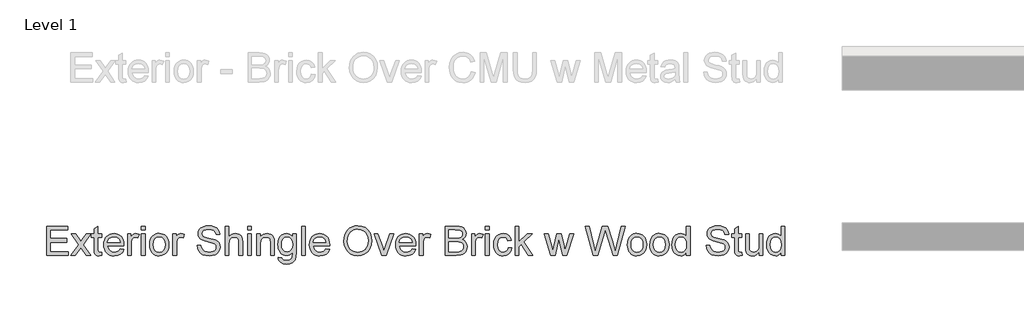
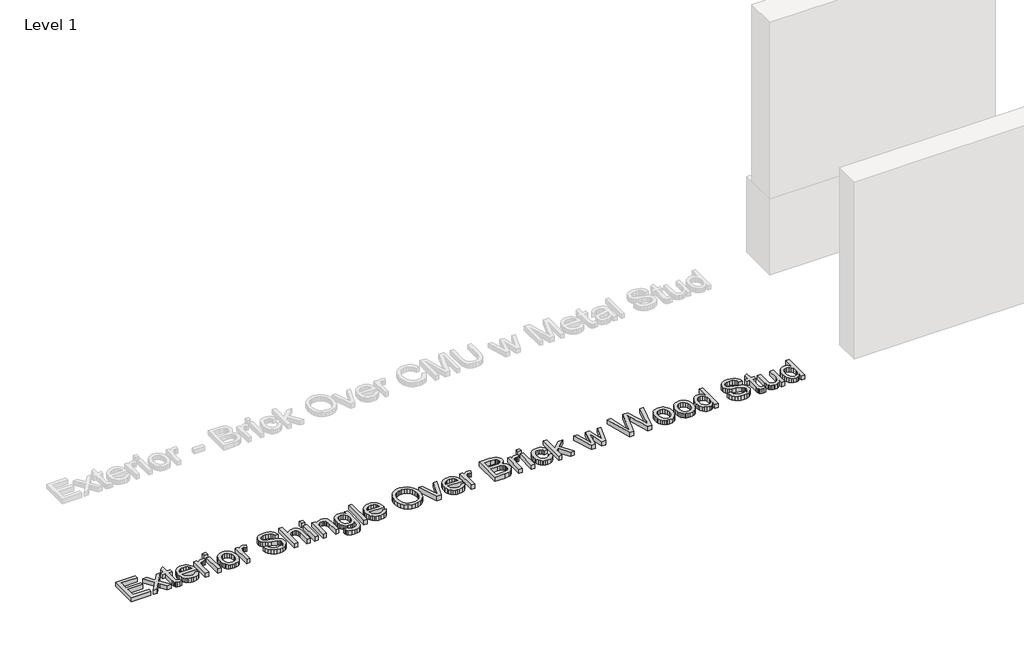
# One storey, part 38 of 42: 1 proxy.
"""IFC4 building model written with IfcOpenShell, lengths in millimetres."""

from ifc_helpers import new_model, si_unit, origin, origin_with_axes, place, context, project, spatial, polyline, outline, extrude, element, save

model = new_model("IFC4")

# Units and contexts
model_context = context("Model", 3, world=origin())
ifc_project = project(units=[si_unit("LENGTHUNIT", "METRE", prefix="MILLI")], contexts=[model_context])

# Site, building, storey
site = spatial("IfcSite", under=ifc_project)
building = spatial("IfcBuilding", under=site)
storey = spatial("IfcBuildingStorey", under=building, Name="Level 1", Elevation=0.0)

# Proxy
placement = place(None, origin())
element("IfcBuildingElementProxy", 1, Name="8\" Arial", ObjectType="8\" Arial", at=placement, inside=storey, context=model_context, shape_type="SweptSolid", body=[
    extrude(outline(polyline([(27228.7881133, 13210.6462247), (27228.7881133, 13515.2133187), (27447.6957121, 13515.2133187), (27447.6957121, 13477.142432), (27266.859, 13477.142432), (27266.859, 13386.7240759), (27438.1779905, 13386.7240759), (27438.1779905, 13348.6531892), (27266.859, 13348.6531892), (27266.859, 13248.7171114), (27452.454573, 13248.7171114), (27452.454573, 13210.6462247), (27228.7881133, 13210.6462247)])), origin_with_axes(), (0.0, 0.0, 1.0), 50.8),
    extrude(outline(polyline([(27481.0077381, 13210.6462247), (27562.3545156, 13323.0743121), (27485.7665989, 13434.3126844), (27531.5706345, 13434.3126844), (27568.5261633, 13380.7754999), (27585.7770338, 13355.4940516), (27600.7228312, 13376.1653534), (27642.8090068, 13434.3126844), (27688.6130424, 13434.3126844), (27608.1585513, 13323.0743121), (27685.6387544, 13210.6462247), (27639.8347188, 13210.6462247), (27593.2127539, 13278.2369201), (27584.6616758, 13290.5802154), (27526.8117737, 13210.6462247), (27481.0077381, 13210.6462247)])), origin_with_axes(), (0.0, 0.0, 1.0), 50.8),
    extrude(outline(polyline([(27799.8514147, 13242.3967494), (27804.6102755, 13209.5308667), (27776.1314676, 13205.8873638), (27757.8581856, 13207.4674543), (27744.2322285, 13212.2077259), (27734.602971, 13219.5133208), (27728.3197876, 13228.7893816), (27724.8621778, 13244.7204119), (27723.7096411, 13271.9909152), (27723.7096411, 13396.2417976), (27695.1564761, 13396.2417976), (27695.1564761, 13434.3126844), (27723.7096411, 13434.3126844), (27723.7096411, 13488.6677981), (27761.7805279, 13511.0493155), (27761.7805279, 13434.3126844), (27799.8514147, 13434.3126844), (27799.8514147, 13396.2417976), (27761.7805279, 13396.2417976), (27761.7805279, 13273.1062732), (27763.7881723, 13253.4759723), (27770.2944274, 13246.523574), (27783.2697589, 13243.9582506), (27799.8514147, 13242.3967494)])), origin_with_axes(), (0.0, 0.0, 1.0), 50.8),
    extrude(outline(polyline([(27994.5185661, 13277.2702765), (28031.8458808, 13272.5114156), (28018.3965222, 13244.3858045), (27996.9351751, 13223.361306), (27967.9451615, 13210.2558494), (27931.9098031, 13205.8873638), (27908.2874499, 13207.7718541), (27887.2397148, 13213.425325), (27868.7665977, 13222.8477766), (27852.8680988, 13236.0392087), (27840.0833076, 13252.6324828), (27830.9513139, 13272.2604601), (27825.4721176, 13294.9231407), (27823.6457189, 13320.6205245), (27825.4907069, 13347.1892818), (27831.0256711, 13370.6071527), (27840.2506113, 13390.8741372), (27853.1655276, 13407.9902353), (27869.0222006, 13421.5883084), (27887.0724111, 13431.3012177), (27907.316159, 13437.1289633), (27929.7534443, 13439.0715452), (27951.4680706, 13437.1336107), (27971.1053425, 13431.319807), (27988.6652602, 13421.6301343), (28004.1478236, 13408.0645925), (28016.786224, 13390.985673), (28025.8136529, 13370.7558671), (28031.2301103, 13347.3751748), (28033.0355961, 13320.8435961), (28032.8125245, 13310.5823024), (27861.7166056, 13310.5823024), (27868.3065126, 13282.0849052), (27883.6148013, 13261.1347639), (27905.7081845, 13248.2523789), (27932.6533751, 13243.9582506), (27952.9157123, 13245.9473057), (27969.9806899, 13251.9144711), (27983.8483078, 13262.2315326), (27994.5185661, 13277.2702765)]), holes=[polyline([(27861.7166056, 13348.6531892), (27994.9647093, 13348.6531892), (27989.8154732, 13368.766812), (27979.7214832, 13383.1549303), (27957.5258587, 13396.5392264), (27929.6047299, 13401.0006585), (27903.942201, 13397.4408075), (27882.7225148, 13386.7612545), (27867.9719052, 13370.1145362), (27861.7166056, 13348.6531892)])]), origin_with_axes(), (0.0, 0.0, 1.0), 50.8),
    extrude(outline(polyline([(28071.1064828, 13210.6462247), (28071.1064828, 13434.3126844), (28104.4185087, 13434.3126844), (28104.4185087, 13401.2237301), (28116.7246254, 13420.4078878), (28128.0640986, 13431.7101823), (28139.4407503, 13437.2312045), (28151.8584028, 13439.0715452), (28170.819489, 13436.1344358), (28190.0780039, 13427.3231075), (28177.3629226, 13393.1931524), (28163.9786265, 13399.0487819), (28150.5943304, 13401.0006585), (28139.2269733, 13399.1231391), (28129.0679208, 13393.4905812), (28120.8607447, 13384.5305385), (28115.3490172, 13372.670565), (28110.7202815, 13351.4044056), (28109.1773696, 13328.204959), (28109.1773696, 13210.6462247), (28071.1064828, 13210.6462247)])), origin_with_axes(), (0.0, 0.0, 1.0), 50.8),
    extrude(outline(polyline([(28213.8723082, 13477.142432), (28213.8723082, 13515.2133187), (28251.9431949, 13515.2133187), (28251.9431949, 13477.142432), (28213.8723082, 13477.142432)])), origin_with_axes(), (0.0, 0.0, 1.0), 50.8),
    extrude(outline(polyline([(28213.8723082, 13210.6462247), (28213.8723082, 13434.3126844), (28251.9431949, 13434.3126844), (28251.9431949, 13210.6462247), (28213.8723082, 13210.6462247)])), origin_with_axes(), (0.0, 0.0, 1.0), 50.8),
    extrude(outline(polyline([(28299.5318034, 13322.4794545), (28301.5905684, 13351.4462315), (28307.7668633, 13376.4070143), (28318.0606883, 13397.3618029), (28332.4720433, 13414.3105974), (28346.9809921, 13425.1435121), (28362.9956742, 13432.8813083), (28380.5160896, 13437.523986), (28399.5422383, 13439.0715452), (28420.5458238, 13437.1870549), (28439.5371176, 13431.533584), (28456.5161197, 13422.1111325), (28471.48283, 13408.9197003), (28483.6983239, 13392.4054308), (28492.4236766, 13373.014467), (28497.6588883, 13350.7468091), (28499.4039589, 13325.6024569), (28496.318135, 13287.1411949), (28487.0606635, 13257.8630471), (28471.9010892, 13235.9369675), (28451.108957, 13219.5319101), (28426.4130717, 13209.2985004), (28399.5422383, 13205.8873638), (28378.2319293, 13207.7648831), (28359.0640372, 13213.3974411), (28342.0385619, 13222.7850377), (28327.1555034, 13235.9276729), (28315.0701347, 13252.6022752), (28306.4377284, 13272.5857728), (28301.2582846, 13295.878166), (28299.5318034, 13322.4794545)]), holes=[polyline([(28337.6026901, 13322.5538117), (28342.0083543, 13288.0985438), (28355.2253467, 13263.551373), (28375.1158979, 13248.8565312), (28399.5422383, 13243.9582506), (28423.8570429, 13248.8844151), (28443.7104155, 13263.6629088), (28456.927408, 13288.5353924), (28461.3330721, 13323.7435269), (28456.899524, 13357.1949726), (28443.5988797, 13381.4075361), (28423.7176232, 13396.1023779), (28399.5422383, 13401.0006585), (28375.1158979, 13396.1209672), (28355.2253467, 13381.4818933), (28342.0083543, 13356.9904903), (28337.6026901, 13322.5538117)])]), origin_with_axes(), (0.0, 0.0, 1.0), 50.8),
    extrude(outline(polyline([(28542.2337065, 13210.6462247), (28542.2337065, 13434.3126844), (28575.5457324, 13434.3126844), (28575.5457324, 13401.2237301), (28587.8518491, 13420.4078878), (28599.1913222, 13431.7101823), (28610.5679739, 13437.2312045), (28622.9856264, 13439.0715452), (28641.9467126, 13436.1344358), (28661.2052276, 13427.3231075), (28648.4901463, 13393.1931524), (28635.1058501, 13399.0487819), (28621.721554, 13401.0006585), (28610.3541969, 13399.1231391), (28600.1951444, 13393.4905812), (28591.9879684, 13384.5305385), (28586.4762409, 13372.670565), (28581.8475051, 13351.4044056), (28580.3045932, 13328.204959), (28580.3045932, 13210.6462247), (28542.2337065, 13210.6462247)])), origin_with_axes(), (0.0, 0.0, 1.0), 50.8),
    extrude(outline(polyline([(28794.4533312, 13315.3411632), (28832.524218, 13315.3411632), (28836.8927035, 13294.2144236), (28844.7931561, 13277.2330979), (28857.1178621, 13263.7558553), (28874.759108, 13253.1413649), (28896.3226962, 13246.2540291), (28920.4144292, 13243.9582506), (28941.6248207, 13245.6963501), (28960.1955316, 13250.9106488), (28975.2435701, 13259.1642981), (28985.8859444, 13270.0204494), (28992.2156011, 13282.4845752), (28994.3254867, 13295.5621479), (28992.7453962, 13308.3051131), (28988.0051247, 13319.3192735), (28978.3758672, 13328.7161647), (28962.1288188, 13336.6073226), (28906.6955257, 13351.1441554), (28870.3069706, 13360.7641182), (28847.0238721, 13369.9193486), (28828.0720806, 13382.7273764), (28814.6413112, 13398.249442), (28806.6386175, 13416.1509381), (28803.9710529, 13436.0972572), (28807.2706537, 13458.3951227), (28817.169456, 13479.187255), (28833.4072097, 13496.8099116), (28855.7236646, 13509.5993501), (28882.5108462, 13517.3789722), (28912.1607799, 13519.9721796), (28944.2830906, 13517.2581417), (28972.3901125, 13509.1160283), (28995.4780233, 13495.7131428), (29012.5430009, 13477.2167892), (29023.3433843, 13454.7795039), (29027.6375126, 13429.5538235), (28989.5666259, 13429.5538235), (28982.577049, 13452.2699483), (28968.0030377, 13468.6657111), (28945.231145, 13478.5923974), (28913.647924, 13481.9012928), (28881.3211309, 13478.629576), (28859.1440958, 13468.8144255), (28846.3174787, 13454.3705393), (28842.0419397, 13437.2126152), (28845.0719956, 13422.582836), (28854.1621634, 13410.8158089), (28875.6513944, 13400.294265), (28916.3247832, 13389.5496495), (28958.299423, 13379.3441238), (28983.692407, 13370.439849), (29005.395415, 13356.6279989), (29020.5364, 13339.5816107), (29029.4313801, 13319.4865772), (29032.3963735, 13296.5287915), (29028.9852369, 13273.0598), (29018.7518271, 13250.985006), (29002.1144035, 13231.9867413), (28979.4912252, 13217.7473373), (28952.2857844, 13208.8523572), (28921.9015732, 13205.8873638), (28884.6021424, 13209.0847234), (28853.9019132, 13218.6768023), (28829.4476888, 13234.7007791), (28810.8862726, 13257.1938323), (28798.9705312, 13284.5944608), (28794.4533312, 13315.3411632)])), origin_with_axes(), (0.0, 0.0, 1.0), 50.8),
    extrude(outline(polyline([(29084.7438428, 13210.6462247), (29084.7438428, 13515.2133187), (29122.8147295, 13515.2133187), (29122.8147295, 13403.2313745), (29136.7985306, 13418.9114492), (29152.5018419, 13430.1115025), (29169.9246635, 13436.8315345), (29189.0669953, 13439.0715452), (29212.0619597, 13436.6270522), (29231.8223858, 13429.2935733), (29247.38163, 13417.6473768), (29257.7730488, 13402.2647309), (29263.6286783, 13381.1286966), (29265.5805549, 13352.2223348), (29265.5805549, 13210.6462247), (29227.5096681, 13210.6462247), (29227.5096681, 13348.2814032), (29224.4796122, 13372.112886), (29215.3894444, 13388.4342915), (29200.7410759, 13397.8590667), (29181.0364177, 13401.0006585), (29164.9473784, 13398.8814782), (29149.843572, 13392.5239376), (29137.332973, 13382.5414834), (29129.0235558, 13369.5475626), (29124.3669361, 13352.2781027), (29122.8147295, 13329.4690314), (29122.8147295, 13210.6462247), (29084.7438428, 13210.6462247)])), origin_with_axes(), (0.0, 0.0, 1.0), 50.8),
    extrude(outline(polyline([(29317.9280242, 13210.6462247), (29317.9280242, 13434.3126844), (29355.9989109, 13434.3126844), (29355.9989109, 13210.6462247), (29317.9280242, 13210.6462247)])), origin_with_axes(), (0.0, 0.0, 1.0), 50.8),
    extrude(outline(polyline([(29317.9280242, 13477.142432), (29317.9280242, 13515.2133187), (29355.9989109, 13515.2133187), (29355.9989109, 13477.142432), (29317.9280242, 13477.142432)])), origin_with_axes(), (0.0, 0.0, 1.0), 50.8),
    extrude(outline(polyline([(29413.1052411, 13210.6462247), (29413.1052411, 13434.3126844), (29451.1761278, 13434.3126844), (29451.1761278, 13403.0826601), (29464.4024149, 13418.8277973), (29480.2869719, 13430.0743239), (29498.8297988, 13436.8222399), (29520.0308957, 13439.0715452), (29538.7967942, 13437.2590884), (29555.9826022, 13431.8217181), (29570.3149526, 13423.4379438), (29580.5204784, 13412.7862748), (29591.9343087, 13384.7907887), (29593.9419532, 13347.9839744), (29593.9419532, 13210.6462247), (29555.8710664, 13210.6462247), (29555.8710664, 13342.8533275), (29551.4839916, 13376.5371394), (29545.4145851, 13386.5660669), (29535.9805152, 13394.345689), (29523.8881755, 13399.3369161), (29509.8439592, 13401.0006585), (29487.5460936, 13397.2642091), (29468.5385342, 13386.0548611), (29460.9424814, 13376.9042781), (29455.5167294, 13364.3983264), (29451.1761278, 13329.320317), (29451.1761278, 13210.6462247), (29413.1052411, 13210.6462247)])), origin_with_axes(), (0.0, 0.0, 1.0), 50.8),
    extrude(outline(polyline([(29636.7717008, 13191.6107813), (29674.8425875, 13186.8519204), (29679.0437694, 13174.9547683), (29687.1858828, 13166.7754762), (29703.1912703, 13160.4179356), (29724.1414116, 13158.2987554), (29746.4857504, 13160.6967751), (29763.1045848, 13167.8908343), (29774.6299509, 13179.4162004), (29781.6938849, 13194.8081409), (29784.296387, 13239.1993897), (29771.6277789, 13226.70738), (29757.4906161, 13217.7845159), (29741.8848986, 13212.4307975), (29724.8106264, 13210.6462247), (29703.937166, 13212.723579), (29685.5593191, 13218.9556418), (29669.6770857, 13229.3424133), (29656.2904659, 13243.8838934), (29645.6690046, 13261.3299516), (29638.0822464, 13280.4304575), (29633.5301915, 13301.1854112), (29632.0128399, 13323.5948125), (29634.7361724, 13354.3322204), (29642.9061698, 13382.5972513), (29656.234698, 13406.5495646), (29674.4336229, 13424.3488195), (29696.8802029, 13435.3908638), (29722.9516964, 13439.0715452), (29740.7555986, 13436.9895436), (29756.9143478, 13430.7435387), (29771.4279439, 13420.3335306), (29784.296387, 13405.7595193), (29784.296387, 13434.3126844), (29822.3672737, 13434.3126844), (29822.3672737, 13241.2070341), (29819.7647717, 13196.6205977), (29811.9572656, 13167.2587981), (29798.5079069, 13147.7865061), (29778.9798471, 13132.8685927), (29753.80064, 13123.3880496), (29723.3978396, 13120.2278686), (29687.9759281, 13124.680006), (29660.0826832, 13138.0364182), (29649.5774049, 13148.063022), (29642.1904818, 13160.3342837), (29637.9219137, 13174.8502035), (29636.7717008, 13191.6107813)]), holes=[polyline([(29670.0837267, 13326.1973145), (29674.1454888, 13291.2773142), (29686.330775, 13267.269233), (29704.6505304, 13253.3551418), (29727.1156996, 13248.7171114), (29749.4135652, 13253.3272579), (29767.826267, 13267.1576972), (29780.178857, 13290.8590549), (29784.296387, 13325.0819565), (29780.0580265, 13358.087259), (29767.3429452, 13381.8536793), (29748.6606985, 13396.2139137), (29726.520842, 13401.0006585), (29704.7806555, 13396.2882709), (29686.5538466, 13382.1511081), (29674.2012567, 13358.7378845), (29670.0837267, 13326.1973145)])]), origin_with_axes(), (0.0, 0.0, 1.0), 50.8),
    extrude(outline(polyline([(29879.4736038, 13210.6462247), (29879.4736038, 13515.2133187), (29917.5444906, 13515.2133187), (29917.5444906, 13210.6462247), (29879.4736038, 13210.6462247)])), origin_with_axes(), (0.0, 0.0, 1.0), 50.8),
    extrude(outline(polyline([(30131.2470854, 13277.2702765), (30168.5744002, 13272.5114156), (30155.1250415, 13244.3858045), (30133.6636944, 13223.361306), (30104.6736808, 13210.2558494), (30068.6383224, 13205.8873638), (30045.0159692, 13207.7718541), (30023.9682341, 13213.425325), (30005.4951171, 13222.8477766), (29989.5966181, 13236.0392087), (29976.8118269, 13252.6324828), (29967.6798332, 13272.2604601), (29962.200637, 13294.9231407), (29960.3742382, 13320.6205245), (29962.2192263, 13347.1892818), (29967.7541904, 13370.6071527), (29976.9791306, 13390.8741372), (29989.8940469, 13407.9902353), (30005.7507199, 13421.5883084), (30023.8009304, 13431.3012177), (30044.0446783, 13437.1289633), (30066.4819636, 13439.0715452), (30088.1965899, 13437.1336107), (30107.8338619, 13431.319807), (30125.3937795, 13421.6301343), (30140.8763429, 13408.0645925), (30153.5147434, 13390.985673), (30162.5421723, 13370.7558671), (30167.9586296, 13347.3751748), (30169.7641154, 13320.8435961), (30169.5410438, 13310.5823024), (29998.445125, 13310.5823024), (30005.0350319, 13282.0849052), (30020.3433206, 13261.1347639), (30042.4367038, 13248.2523789), (30069.3818944, 13243.9582506), (30089.6442316, 13245.9473057), (30106.7092092, 13251.9144711), (30120.5768271, 13262.2315326), (30131.2470854, 13277.2702765)]), holes=[polyline([(29998.445125, 13348.6531892), (30131.6932286, 13348.6531892), (30126.5439925, 13368.766812), (30116.4500025, 13383.1549303), (30094.2543781, 13396.5392264), (30066.3332492, 13401.0006585), (30040.6707203, 13397.4408075), (30019.4510342, 13386.7612545), (30004.7004245, 13370.1145362), (29998.445125, 13348.6531892)])]), origin_with_axes(), (0.0, 0.0, 1.0), 50.8),
    extrude(outline(polyline([(30317.2888016, 13358.9144829), (30319.826241, 13394.6384705), (30327.4385595, 13426.2635174), (30340.1257568, 13453.7896236), (30357.8878332, 13477.2167892), (30379.660551, 13495.9222725), (30404.3796729, 13509.283332), (30432.0451989, 13517.2999677), (30462.6571289, 13519.9721796), (30502.605535, 13514.9530685), (30538.4271165, 13499.8957354), (30568.1699967, 13475.8597703), (30589.8822993, 13443.9047633), (30603.1550597, 13405.5736263), (30607.5793131, 13362.4092713), (30602.9226934, 13318.668648), (30588.9528343, 13279.7984213), (30566.4411918, 13247.7876464), (30536.1592218, 13224.6253784), (30500.6443638, 13210.5718675), (30462.4340573, 13205.8873638), (30421.8722044, 13211.0644839), (30385.8461406, 13226.5958442), (30356.1776175, 13251.0779525), (30334.6883865, 13283.1073167), (30321.6386978, 13319.9606043), (30317.2888016, 13358.9144829)]), holes=[polyline([(30355.3596883, 13358.5426969), (30357.2627679, 13333.3030745), (30362.9720068, 13310.8983205), (30372.4874048, 13291.3284347), (30385.808962, 13274.5934173), (30402.0025661, 13261.1905318), (30420.1341048, 13251.6170422), (30440.203578, 13245.8729485), (30462.2109857, 13243.9582506), (30484.5948268, 13245.8915378), (30504.9013136, 13251.6913994), (30523.1304461, 13261.3578355), (30539.2822243, 13274.8908461), (30552.5061877, 13291.9790603), (30561.9518758, 13312.3111073), (30567.6192887, 13335.8869873), (30569.5084263, 13362.7067001), (30566.2738881, 13396.4091013), (30556.5702734, 13425.5385347), (30540.6485378, 13449.3607229), (30518.7596369, 13467.1413885), (30492.353536, 13478.2113167), (30462.8802005, 13481.9012928), (30441.6372778, 13480.123691), (30421.9279723, 13474.7908855), (30403.752284, 13465.9028764), (30387.110213, 13453.4596635), (30373.2193585, 13436.8617422), (30363.2973195, 13415.5096072), (30357.3440961, 13389.4032588), (30355.3596883, 13358.5426969)])]), origin_with_axes(), (0.0, 0.0, 1.0), 50.8),
    extrude(outline(polyline([(30710.0435357, 13210.6462247), (30631.3736173, 13434.3126844), (30671.6752201, 13434.3126844), (30719.3381858, 13300.3210087), (30733.6891255, 13255.2605451), (30747.7426364, 13297.7928639), (30795.7030309, 13434.3126844), (30836.0046337, 13434.3126844), (30758.3013589, 13210.6462247), (30710.0435357, 13210.6462247)])), origin_with_axes(), (0.0, 0.0, 1.0), 50.8),
    extrude(outline(polyline([(31025.9129242, 13277.2702765), (31063.240239, 13272.5114156), (31049.7908803, 13244.3858045), (31028.3295333, 13223.361306), (30999.3395196, 13210.2558494), (30963.3041613, 13205.8873638), (30939.6818081, 13207.7718541), (30918.6340729, 13213.425325), (30900.1609559, 13222.8477766), (30884.2624569, 13236.0392087), (30871.4776657, 13252.6324828), (30862.345672, 13272.2604601), (30856.8664758, 13294.9231407), (30855.040077, 13320.6205245), (30856.8850651, 13347.1892818), (30862.4200292, 13370.6071527), (30871.6449694, 13390.8741372), (30884.5598857, 13407.9902353), (30900.4165588, 13421.5883084), (30918.4667692, 13431.3012177), (30938.7105171, 13437.1289633), (30961.1478024, 13439.0715452), (30982.8624287, 13437.1336107), (31002.4997007, 13431.319807), (31020.0596184, 13421.6301343), (31035.5421817, 13408.0645925), (31048.1805822, 13390.985673), (31057.2080111, 13370.7558671), (31062.6244684, 13347.3751748), (31064.4299542, 13320.8435961), (31064.2068826, 13310.5823024), (30893.1109638, 13310.5823024), (30899.7008707, 13282.0849052), (30915.0091594, 13261.1347639), (30937.1025427, 13248.2523789), (30964.0477333, 13243.9582506), (30984.3100705, 13245.9473057), (31001.375048, 13251.9144711), (31015.2426659, 13262.2315326), (31025.9129242, 13277.2702765)]), holes=[polyline([(30893.1109638, 13348.6531892), (31026.3590675, 13348.6531892), (31021.2098313, 13368.766812), (31011.1158413, 13383.1549303), (30988.9202169, 13396.5392264), (30960.999088, 13401.0006585), (30935.3365591, 13397.4408075), (30914.116873, 13386.7612545), (30899.3662633, 13370.1145362), (30893.1109638, 13348.6531892)])]), origin_with_axes(), (0.0, 0.0, 1.0), 50.8),
    extrude(outline(polyline([(31102.500841, 13210.6462247), (31102.500841, 13434.3126844), (31135.8128669, 13434.3126844), (31135.8128669, 13401.2237301), (31148.1189836, 13420.4078878), (31159.4584567, 13431.7101823), (31170.8351084, 13437.2312045), (31183.2527609, 13439.0715452), (31202.2138471, 13436.1344358), (31221.4723621, 13427.3231075), (31208.7572808, 13393.1931524), (31195.3729846, 13399.0487819), (31181.9886885, 13401.0006585), (31170.6213315, 13399.1231391), (31160.4622789, 13393.4905812), (31152.2551029, 13384.5305385), (31146.7433754, 13372.670565), (31142.1146396, 13351.4044056), (31140.5717277, 13328.204959), (31140.5717277, 13210.6462247), (31102.500841, 13210.6462247)])), origin_with_axes(), (0.0, 0.0, 1.0), 50.8),
    extrude(outline(polyline([(31368.9970483, 13210.6462247), (31368.9970483, 13515.2133187), (31485.217353, 13515.2133187), (31517.1816546, 13512.9733081), (31542.1377901, 13506.253276), (31561.26618, 13494.885919), (31575.7472448, 13478.7039332), (31584.8652966, 13459.6684898), (31587.9046471, 13439.74076), (31585.3486184, 13421.4024154), (31577.680532, 13404.1608395), (31564.8446203, 13389.0756224), (31546.7851152, 13377.2063542), (31568.357998, 13365.9412383), (31584.2983229, 13348.8019036), (31594.1413573, 13326.9222973), (31597.4223688, 13301.4363667), (31595.1823582, 13280.1980913), (31588.4623261, 13260.5027277), (31578.4333987, 13243.7537683), (31566.2667017, 13231.3547051), (31551.3673776, 13222.3760731), (31533.1405688, 13215.8884073), (31484.3250666, 13210.6462247), (31368.9970483, 13210.6462247)]), holes=[polyline([(31407.067935, 13391.4829368), (31476.5919177, 13391.4829368), (31517.1909493, 13394.7546536), (31531.4024693, 13400.3965062), (31541.6172897, 13408.8453431), (31547.7796427, 13419.9710393), (31549.8337604, 13433.6434696), (31547.9190625, 13446.9162299), (31542.1749687, 13458.4787746), (31532.8617293, 13467.5038798), (31520.2395945, 13473.1643217), (31471.3125564, 13477.142432), (31407.067935, 13477.142432), (31407.067935, 13391.4829368)]), polyline([(31407.067935, 13248.7171114), (31485.1429958, 13248.7171114), (31513.398732, 13250.2042554), (31537.3045721, 13258.4950833), (31553.1426558, 13275.4113465), (31557.7992755, 13287.3642665), (31559.3514821, 13301.0645807), (31557.5297307, 13316.9770217), (31552.0644764, 13330.6587466), (31542.5188708, 13341.3568888), (31528.4560652, 13348.3185818), (31508.53763, 13352.1386829), (31481.4251357, 13353.41205), (31407.067935, 13353.41205), (31407.067935, 13248.7171114)])]), origin_with_axes(), (0.0, 0.0, 1.0), 50.8),
    extrude(outline(polyline([(31645.0109773, 13210.6462247), (31645.0109773, 13434.3126844), (31678.3230032, 13434.3126844), (31678.3230032, 13401.2237301), (31690.6291199, 13420.4078878), (31701.968593, 13431.7101823), (31713.3452447, 13437.2312045), (31725.7628972, 13439.0715452), (31744.7239834, 13436.1344358), (31763.9824984, 13427.3231075), (31751.2674171, 13393.1931524), (31737.883121, 13399.0487819), (31724.4988248, 13401.0006585), (31713.1314678, 13399.1231391), (31702.9724152, 13393.4905812), (31694.7652392, 13384.5305385), (31689.2535117, 13372.670565), (31684.6247759, 13351.4044056), (31683.081864, 13328.204959), (31683.081864, 13210.6462247), (31645.0109773, 13210.6462247)])), origin_with_axes(), (0.0, 0.0, 1.0), 50.8),
    extrude(outline(polyline([(31787.7768026, 13477.142432), (31787.7768026, 13515.2133187), (31825.8476894, 13515.2133187), (31825.8476894, 13477.142432), (31787.7768026, 13477.142432)])), origin_with_axes(), (0.0, 0.0, 1.0), 50.8),
    extrude(outline(polyline([(31787.7768026, 13210.6462247), (31787.7768026, 13434.3126844), (31825.8476894, 13434.3126844), (31825.8476894, 13210.6462247), (31787.7768026, 13210.6462247)])), origin_with_axes(), (0.0, 0.0, 1.0), 50.8),
    extrude(outline(polyline([(32025.7198449, 13291.546859), (32063.7907316, 13286.7879982), (32053.1762412, 13252.9275879), (32033.2299221, 13227.3394162), (32005.8292937, 13211.2503769), (31972.8518752, 13205.8873638), (31951.4997403, 13207.7579121), (31932.3550847, 13213.3695571), (31915.4179086, 13222.7222988), (31900.6882119, 13235.8161371), (31888.7654995, 13252.4047638), (31880.2492763, 13272.2418708), (31875.1395425, 13295.3274579), (31873.4362978, 13321.6615253), (31876.3455233, 13355.5405249), (31885.0731997, 13384.9023245), (31899.7587469, 13408.6129769), (31920.5415845, 13425.5385347), (31945.4047735, 13435.6882926), (31972.3313748, 13439.0715452), (32004.5001587, 13434.4242202), (32030.2184555, 13420.482245), (32048.6683359, 13397.9891918), (32059.0318708, 13367.6886325), (32020.960984, 13362.9297717), (32014.055059, 13379.5393114), (32003.3011489, 13391.4457582), (31989.2941112, 13398.6119334), (31972.6288036, 13401.0006585), (31948.0258648, 13396.2975655), (31928.4978049, 13382.1882867), (31915.7548397, 13357.9106606), (31911.5071846, 13322.7025261), (31915.6618932, 13287.0203644), (31928.1260189, 13262.6590866), (31947.3008821, 13248.6334596), (31971.5878028, 13243.9582506), (31991.3017556, 13246.8767707), (32007.4651521, 13255.6323311), (32019.2228845, 13270.4480033), (32025.7198449, 13291.546859)])), origin_with_axes(), (0.0, 0.0, 1.0), 50.8),
    extrude(outline(polyline([(32097.1027575, 13210.6462247), (32097.1027575, 13515.2133187), (32135.1736443, 13515.2133187), (32135.1736443, 13351.55312), (32220.5357107, 13434.3126844), (32273.1806088, 13434.3126844), (32186.7775416, 13350.5121192), (32277.9394696, 13210.6462247), (32233.4738636, 13210.6462247), (32159.4884489, 13324.0409557), (32135.1736443, 13300.4697231), (32135.1736443, 13210.6462247), (32097.1027575, 13210.6462247)])), origin_with_axes(), (0.0, 0.0, 1.0), 50.8),
    extrude(outline(polyline([(32467.3272598, 13210.6462247), (32399.2904212, 13434.3126844), (32438.848452, 13434.3126844), (32477.4398391, 13303.8157971), (32488.9652052, 13257.1938323), (32498.4085697, 13302.1055815), (32529.1180936, 13434.3126844), (32574.475986, 13434.3126844), (32605.0367955, 13302.4773675), (32613.4391592, 13261.8039787), (32625.4850257, 13304.7080835), (32664.1507701, 13434.3126844), (32703.8575152, 13434.3126844), (32635.3001762, 13210.6462247), (32589.273069, 13210.6462247), (32560.0506891, 13341.8123267), (32551.5739682, 13382.7087871), (32513.8748675, 13210.6462247), (32467.3272598, 13210.6462247)])), origin_with_axes(), (0.0, 0.0, 1.0), 50.8),
    extrude(outline(polyline([(32908.26546, 13210.6462247), (32825.2084668, 13515.2133187), (32864.4690688, 13515.2133187), (32912.6525348, 13315.0437344), (32927.523975, 13253.2529007), (32943.4364159, 13307.9054432), (33003.8144629, 13515.2133187), (33060.4002926, 13515.2133187), (33104.271041, 13364.9374161), (33123.0648235, 13309.1695156), (33136.9138521, 13253.2529007), (33151.3391491, 13313.2591616), (33199.9687583, 13515.2133187), (33239.2293603, 13515.2133187), (33156.0980099, 13210.6462247), (33115.4246211, 13210.6462247), (33042.40585, 13445.6149789), (33032.2189135, 13478.4065044), (33020.7679046, 13438.9228308), (32954.21821, 13210.6462247), (32908.26546, 13210.6462247)])), origin_with_axes(), (0.0, 0.0, 1.0), 50.8),
    extrude(outline(polyline([(33263.0236645, 13322.4794545), (33265.0824295, 13351.4462315), (33271.2587245, 13376.4070143), (33281.5525495, 13397.3618029), (33295.9639044, 13414.3105974), (33310.4728532, 13425.1435121), (33326.4875353, 13432.8813083), (33344.0079507, 13437.523986), (33363.0340995, 13439.0715452), (33384.037685, 13437.1870549), (33403.0289788, 13431.533584), (33420.0079808, 13422.1111325), (33434.9746911, 13408.9197003), (33447.190185, 13392.4054308), (33455.9155378, 13373.014467), (33461.1507494, 13350.7468091), (33462.89582, 13325.6024569), (33459.8099962, 13287.1411949), (33450.5525247, 13257.8630471), (33435.3929504, 13235.9369675), (33414.6008181, 13219.5319101), (33389.9049329, 13209.2985004), (33363.0340995, 13205.8873638), (33341.7237905, 13207.7648831), (33322.5558983, 13213.3974411), (33305.530423, 13222.7850377), (33290.6473646, 13235.9276729), (33278.5619958, 13252.6022752), (33269.9295895, 13272.5857728), (33264.7501458, 13295.878166), (33263.0236645, 13322.4794545)]), holes=[polyline([(33301.0945513, 13322.5538117), (33305.5002154, 13288.0985438), (33318.7172078, 13263.551373), (33338.607759, 13248.8565312), (33363.0340995, 13243.9582506), (33387.3489041, 13248.8844151), (33407.2022767, 13263.6629088), (33420.4192691, 13288.5353924), (33424.8249332, 13323.7435269), (33420.3913851, 13357.1949726), (33407.0907409, 13381.4075361), (33387.2094843, 13396.1023779), (33363.0340995, 13401.0006585), (33338.607759, 13396.1209672), (33318.7172078, 13381.4818933), (33305.5002154, 13356.9904903), (33301.0945513, 13322.5538117)])]), origin_with_axes(), (0.0, 0.0, 1.0), 50.8),
    extrude(outline(polyline([(33496.2078459, 13322.4794545), (33498.2666109, 13351.4462315), (33504.4429059, 13376.4070143), (33514.7367309, 13397.3618029), (33529.1480858, 13414.3105974), (33543.6570346, 13425.1435121), (33559.6717167, 13432.8813083), (33577.1921321, 13437.523986), (33596.2182809, 13439.0715452), (33617.2218664, 13437.1870549), (33636.2131602, 13431.533584), (33653.1921622, 13422.1111325), (33668.1588725, 13408.9197003), (33680.3743664, 13392.4054308), (33689.0997192, 13373.014467), (33694.3349308, 13350.7468091), (33696.0800014, 13325.6024569), (33692.9941776, 13287.1411949), (33683.7367061, 13257.8630471), (33668.5771318, 13235.9369675), (33647.7849995, 13219.5319101), (33623.0891143, 13209.2985004), (33596.2182809, 13205.8873638), (33574.9079719, 13207.7648831), (33555.7400797, 13213.3974411), (33538.7146044, 13222.7850377), (33523.831546, 13235.9276729), (33511.7461772, 13252.6022752), (33503.1137709, 13272.5857728), (33497.9343272, 13295.878166), (33496.2078459, 13322.4794545)]), holes=[polyline([(33534.2787327, 13322.5538117), (33538.6843968, 13288.0985438), (33551.9013892, 13263.551373), (33571.7919404, 13248.8565312), (33596.2182809, 13243.9582506), (33620.5330855, 13248.8844151), (33640.3864581, 13263.6629088), (33653.6034505, 13288.5353924), (33658.0091146, 13323.7435269), (33653.5755665, 13357.1949726), (33640.2749223, 13381.4075361), (33620.3936657, 13396.1023779), (33596.2182809, 13401.0006585), (33571.7919404, 13396.1209672), (33551.9013892, 13381.4818933), (33538.6843968, 13356.9904903), (33534.2787327, 13322.5538117)])]), origin_with_axes(), (0.0, 0.0, 1.0), 50.8),
    extrude(outline(polyline([(33876.9167135, 13210.6462247), (33876.9167135, 13246.5607526), (33865.5261198, 13228.766145), (33851.7282118, 13216.055711), (33835.5229893, 13208.4294506), (33816.9104525, 13205.8873638), (33792.2982191, 13209.5680453), (33769.7679873, 13220.6100896), (33750.6953653, 13238.2420408), (33736.4559614, 13261.6924429), (33727.5888652, 13290.0132418), (33724.6331665, 13322.2563829), (33727.3564989, 13354.0998541), (33735.5264964, 13382.8575015), (33749.1338641, 13406.8934666), (33768.1693075, 13424.5718911), (33791.1921557, 13435.4466317), (33816.7617381, 13439.0715452), (33835.3882169, 13436.4783378), (33851.8583369, 13428.6987157), (33865.8189013, 13416.7736797), (33876.9167135, 13401.7442305), (33876.9167135, 13515.2133187), (33914.9876003, 13515.2133187), (33914.9876003, 13210.6462247), (33876.9167135, 13210.6462247)]), holes=[polyline([(33762.7040532, 13322.4050973), (33766.9981816, 13287.9684187), (33779.8805666, 13263.4770158), (33798.5999919, 13248.8379419), (33820.405241, 13243.9582506), (33842.2011954, 13248.6148703), (33860.4465935, 13262.5847294), (33872.7991835, 13286.128078), (33876.9167135, 13319.5051665), (33872.7248263, 13355.9959627), (33860.1491647, 13381.2960003), (33841.4390341, 13396.0744939), (33818.8437397, 13401.0006585), (33796.815419, 13396.2696816), (33778.7652086, 13382.0767509), (33766.7193421, 13357.6968837), (33762.7040532, 13322.4050973)])]), origin_with_axes(), (0.0, 0.0, 1.0), 50.8),
    extrude(outline(polyline([(34081.5477298, 13315.3411632), (34119.6186166, 13315.3411632), (34123.9871021, 13294.2144236), (34131.8875547, 13277.2330979), (34144.2122607, 13263.7558553), (34161.8535066, 13253.1413649), (34183.4170948, 13246.2540291), (34207.5088278, 13243.9582506), (34228.7192193, 13245.6963501), (34247.2899302, 13250.9106488), (34262.3379687, 13259.1642981), (34272.980343, 13270.0204494), (34279.3099997, 13282.4845752), (34281.4198853, 13295.5621479), (34279.8397948, 13308.3051131), (34275.0995232, 13319.3192735), (34265.4702658, 13328.7161647), (34249.2232174, 13336.6073226), (34193.7899243, 13351.1441554), (34157.4013692, 13360.7641182), (34134.1182707, 13369.9193486), (34115.1664792, 13382.7273764), (34101.7357098, 13398.249442), (34093.7330161, 13416.1509381), (34091.0654515, 13436.0972572), (34094.3650523, 13458.3951227), (34104.2638546, 13479.187255), (34120.5016083, 13496.8099116), (34142.8180632, 13509.5993501), (34169.6052448, 13517.3789722), (34199.2551785, 13519.9721796), (34231.3774892, 13517.2581417), (34259.4845111, 13509.1160283), (34282.5724219, 13495.7131428), (34299.6373995, 13477.2167892), (34310.4377829, 13454.7795039), (34314.7319112, 13429.5538235), (34276.6610245, 13429.5538235), (34269.6714476, 13452.2699483), (34255.0974363, 13468.6657111), (34232.3255435, 13478.5923974), (34200.7423225, 13481.9012928), (34168.4155295, 13478.629576), (34146.2384944, 13468.8144255), (34133.4118773, 13454.3705393), (34129.1363383, 13437.2126152), (34132.1663942, 13422.582836), (34141.256562, 13410.8158089), (34162.745793, 13400.294265), (34203.4191818, 13389.5496495), (34245.3938216, 13379.3441238), (34270.7868056, 13370.439849), (34292.4898136, 13356.6279989), (34307.6307986, 13339.5816107), (34316.5257787, 13319.4865772), (34319.4907721, 13296.5287915), (34316.0796355, 13273.0598), (34305.8462257, 13250.985006), (34289.2088021, 13231.9867413), (34266.5856238, 13217.7473373), (34239.380183, 13208.8523572), (34208.9959718, 13205.8873638), (34171.696541, 13209.0847234), (34140.9963118, 13218.6768023), (34116.5420874, 13234.7007791), (34097.9806712, 13257.1938323), (34086.0649298, 13284.5944608), (34081.5477298, 13315.3411632)])), origin_with_axes(), (0.0, 0.0, 1.0), 50.8),
    extrude(outline(polyline([(34452.7388757, 13242.3967494), (34457.4977366, 13209.5308667), (34429.0189287, 13205.8873638), (34410.7456466, 13207.4674543), (34397.1196896, 13212.2077259), (34387.4904321, 13219.5133208), (34381.2072486, 13228.7893816), (34377.7496388, 13244.7204119), (34376.5971022, 13271.9909152), (34376.5971022, 13396.2417976), (34348.0439371, 13396.2417976), (34348.0439371, 13434.3126844), (34376.5971022, 13434.3126844), (34376.5971022, 13488.6677981), (34414.667989, 13511.0493155), (34414.667989, 13434.3126844), (34452.7388757, 13434.3126844), (34452.7388757, 13396.2417976), (34414.667989, 13396.2417976), (34414.667989, 13273.1062732), (34416.6756334, 13253.4759723), (34423.1818884, 13246.523574), (34436.15722, 13243.9582506), (34452.7388757, 13242.3967494)])), origin_with_axes(), (0.0, 0.0, 1.0), 50.8),
    extrude(outline(polyline([(34633.5755878, 13210.6462247), (34633.5755878, 13249.0888974), (34619.8009164, 13230.1882265), (34603.7583503, 13216.6877472), (34585.4478897, 13208.5874597), (34564.8695344, 13205.8873638), (34546.3267075, 13207.7834724), (34529.0665422, 13213.4717983), (34514.5854774, 13222.0228764), (34504.3799516, 13232.5072417), (34497.5112052, 13245.2409123), (34493.0404785, 13260.5399063), (34490.8097625, 13295.9339339), (34490.8097625, 13434.3126844), (34528.8806492, 13434.3126844), (34528.8806492, 13313.8540192), (34531.1857225, 13275.0395605), (34536.7346286, 13262.0921129), (34546.2430556, 13252.2490785), (34559.0789674, 13246.0309575), (34574.6103277, 13243.9582506), (34591.0339744, 13246.0774308), (34606.398031, 13252.4349715), (34619.066639, 13262.4453096), (34627.4039402, 13275.5228823), (34632.0326759, 13293.433673), (34633.5755878, 13317.9436653), (34633.5755878, 13434.3126844), (34671.6464746, 13434.3126844), (34671.6464746, 13210.6462247), (34633.5755878, 13210.6462247)])), origin_with_axes(), (0.0, 0.0, 1.0), 50.8),
    extrude(outline(polyline([(34862.0009084, 13210.6462247), (34862.0009084, 13246.5607526), (34850.6103147, 13228.766145), (34836.8124066, 13216.055711), (34820.6071842, 13208.4294506), (34801.9946474, 13205.8873638), (34777.382414, 13209.5680453), (34754.8521822, 13220.6100896), (34735.7795602, 13238.2420408), (34721.5401563, 13261.6924429), (34712.6730601, 13290.0132418), (34709.7173613, 13322.2563829), (34712.4406938, 13354.0998541), (34720.6106912, 13382.8575015), (34734.218059, 13406.8934666), (34753.2535023, 13424.5718911), (34776.2763506, 13435.4466317), (34801.845933, 13439.0715452), (34820.4724118, 13436.4783378), (34836.9425317, 13428.6987157), (34850.9030962, 13416.7736797), (34862.0009084, 13401.7442305), (34862.0009084, 13515.2133187), (34900.0717951, 13515.2133187), (34900.0717951, 13210.6462247), (34862.0009084, 13210.6462247)]), holes=[polyline([(34747.7882481, 13322.4050973), (34752.0823764, 13287.9684187), (34764.9647615, 13263.4770158), (34783.6841867, 13248.8379419), (34805.4894358, 13243.9582506), (34827.2853903, 13248.6148703), (34845.5307884, 13262.5847294), (34857.8833784, 13286.128078), (34862.0009084, 13319.5051665), (34857.8090212, 13355.9959627), (34845.2333596, 13381.2960003), (34826.523229, 13396.0744939), (34803.9279346, 13401.0006585), (34781.8996139, 13396.2696816), (34763.8494034, 13382.0767509), (34751.8035369, 13357.6968837), (34747.7882481, 13322.4050973)])]), origin_with_axes(), (0.0, 0.0, 1.0), 50.8),
])

save(model, "model.ifc")

# Revit data of these elements
# Element 1 (IfcBuildingElementProxy, "8\" Arial")
#   Phase Created = New Construction
